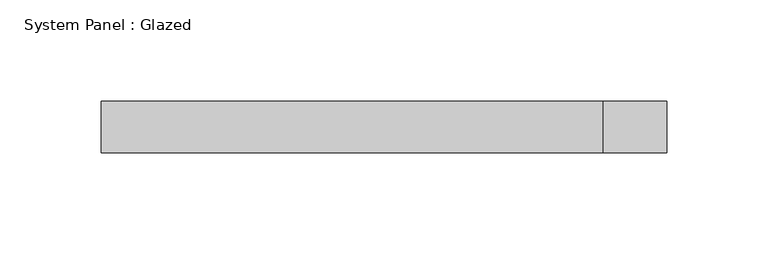
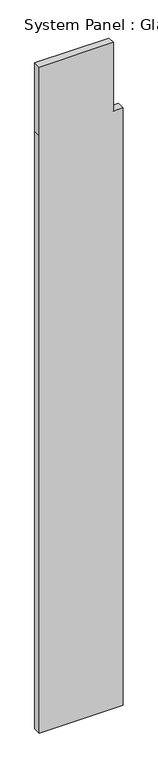
"""IFC4 building model written with IfcOpenShell, lengths in millimetres: plate geometry, System Panel : Glazed."""

from ifc_helpers import new_model, si_unit, frame, origin, place, context, project, spatial, polyline, outline, extrude, source, transform, mapped, element, save


def system_panel_glazed_b71afb28(model_context):
    return source(origin(), model_context, "Body", "SweptSolid", [
        extrude(outline(polyline([(0.0, -139.7), (0.0, 139.7), (2101.85, 139.7), (2101.85, 107.95), (2343.15, 107.95), (2343.15, -139.7), (2101.85, -139.7), (0.0, -139.7)])), frame((0.0, -44.45, 0.0), z_axis=(0.0, 1.0, 0.0), x_axis=(0.0, 0.0, 1.0)), (0.0, 0.0, 1.0), 25.4),
    ])


if __name__ == "__main__":
    model = new_model("IFC4")
    model_context = context("Model", 3, world=origin())
    ifc_project = project(units=[si_unit("LENGTHUNIT", "METRE", prefix="MILLI")], contexts=[model_context])
    site = spatial("IfcSite", under=ifc_project)
    building = spatial("IfcBuilding", under=site)
    placement = place(None, origin())
    system_panel_glazed_shape = system_panel_glazed_b71afb28(model_context)
    element("IfcPlate", 1, ObjectType="System Panel : Glazed", at=placement, inside=building, context=model_context, shape_type="MappedRepresentation", body=[
        mapped(system_panel_glazed_shape, transform((0.0, 0.0, 0.0), x_axis=(1.0, 0.0, 0.0), y_axis=(0.0, 1.0, 0.0), z_axis=(0.0, 0.0, 1.0))),
    ])
    save(model, "model.ifc")

# Revit data of these elements
# Element 1 (IfcPlate, "System Panel : Glazed")
#   Materials on its faces: "Glass"
# Materials
#   "Glass": class "Glass", colour RGB 0 128 192, transparency 0.75, Cost = 0
